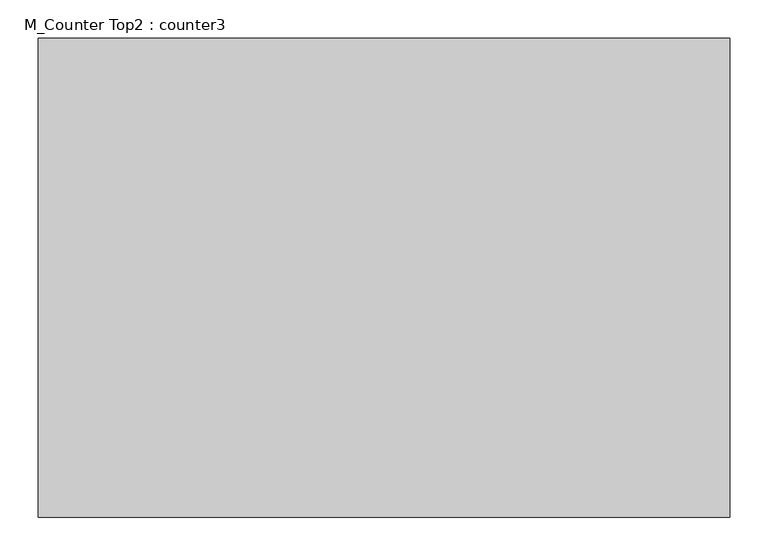
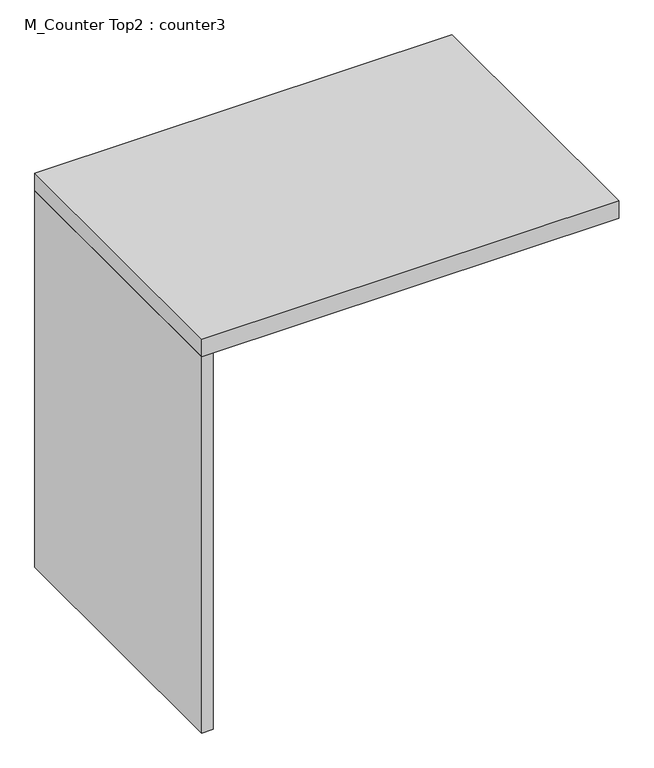
"""IFC4 building model written with IfcOpenShell, lengths in millimetres: furniture geometry, M_Counter Top2 : counter3."""

from ifc_helpers import new_model, si_unit, frame, origin, origin_with_axes, place, context, project, spatial, polyline, outline, extrude, source, transform, mapped, element, save


def m_counter_top2_counter3_b5257813(model_context):
    return source(origin(), model_context, "Body", "SweptSolid", [
        extrude(outline(polyline([(-298.5907219, 0.0), (-298.5907219, -625.0), (-1200.4622951, -625.0), (-1200.4622951, 0.0), (-298.5907219, 0.0)])), frame((0.0, 0.0, 860.0), z_axis=(0.0, 0.0, 1.0), x_axis=(1.0, 0.0, 0.0)), (0.0, 0.0, 1.0), 40.0),
        extrude(outline(polyline([(-1175.4622951, 0.0), (-1175.4622951, -625.0), (-1200.4622951, -625.0), (-1200.4622951, 0.0), (-1175.4622951, 0.0)])), origin_with_axes(), (0.0, 0.0, 1.0), 860.0),
    ])


if __name__ == "__main__":
    model = new_model("IFC4")
    model_context = context("Model", 3, world=origin())
    ifc_project = project(units=[si_unit("LENGTHUNIT", "METRE", prefix="MILLI")], contexts=[model_context])
    site = spatial("IfcSite", under=ifc_project)
    building = spatial("IfcBuilding", under=site)
    placement = place(None, origin())
    m_counter_top2_counter3_shape = m_counter_top2_counter3_b5257813(model_context)
    element("IfcFurniture", 1, ObjectType="M_Counter Top2 : counter3", at=placement, inside=building, context=model_context, shape_type="MappedRepresentation", body=[
        mapped(m_counter_top2_counter3_shape, transform((0.0, 0.0, 0.0), x_axis=(1.0, 0.0, 0.0), y_axis=(0.0, 1.0, 0.0), z_axis=(0.0, 0.0, 1.0))),
    ])
    save(model, "model.ifc")

# Revit data of these elements
# Type "M_Counter Top2 : counter3"
#   Counter Thickness = 0' - 1.5748"
#   Depth = 2' - 0.6063"
#   Height = 2' - 11.43307"
#   Length [instance default] = 8' - 2.4252"
#   Counter Top Material = Counter Top
#   Default Elevation = 0
# Element 1 (IfcFurniture, "M_Counter Top2 : counter3")
#   Length = 2' - 11.50675"
#   Materials on its faces: "Counter Top"
# Materials
#   "Counter Top": class "Wood", colour RGB 226 177 128, transparency 0
